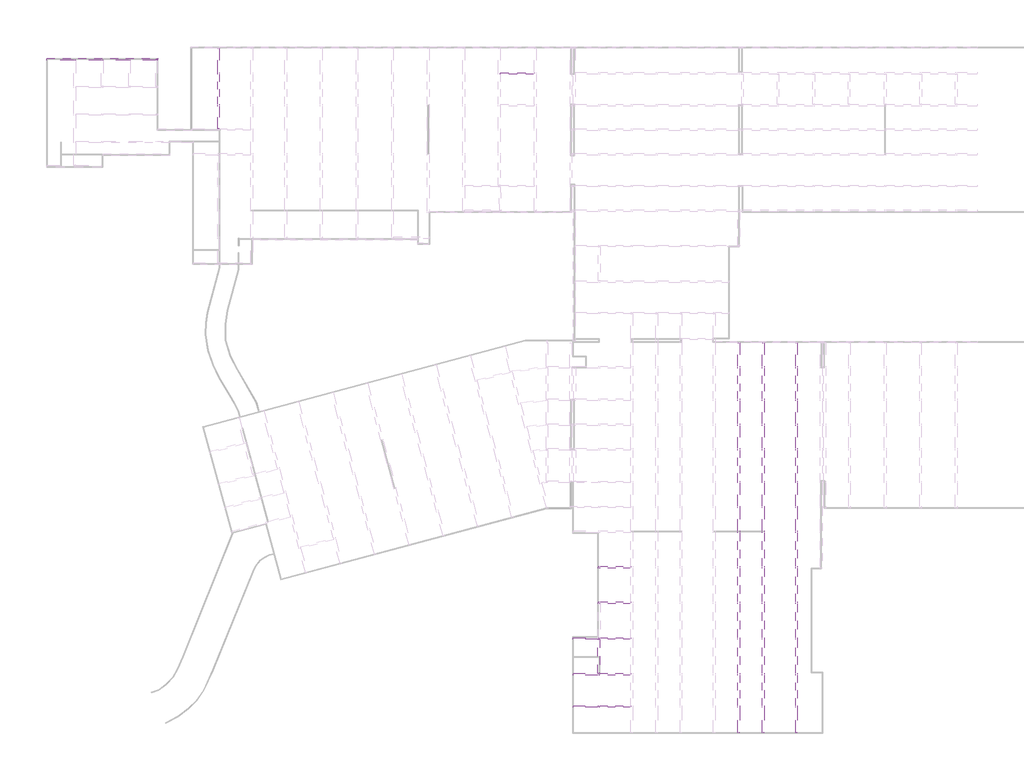
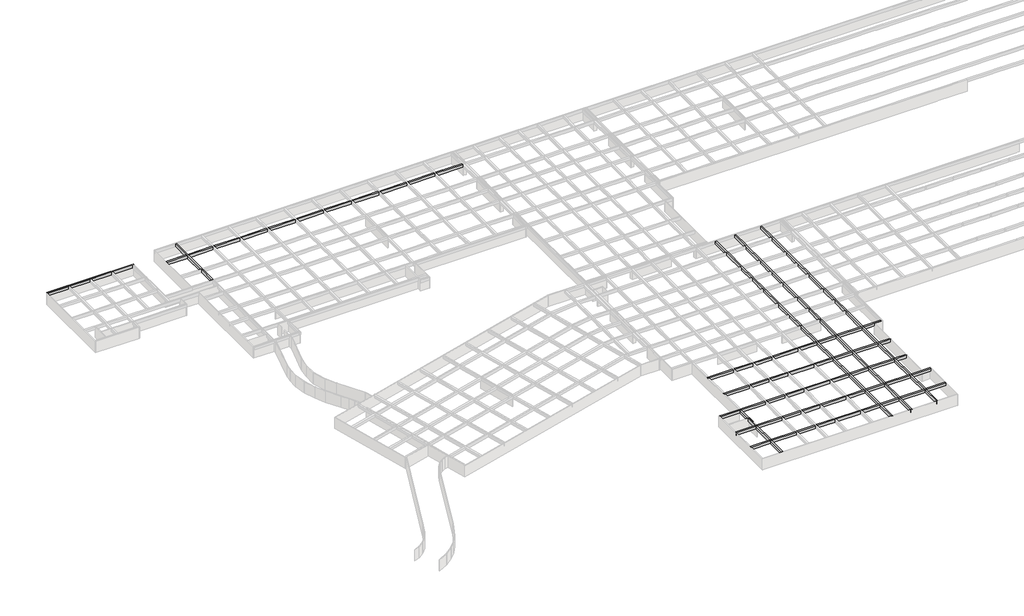
# One storey, part 6 of 14: 12 beams.
"""IFC4 building model written with IfcOpenShell, lengths in millimetres."""

import ifcopenshell
import ifcopenshell.guid

model = None  # the IFC model being written
_history = None  # IfcOwnerHistory: only IFC2X3 demands one
_inside = {}  # id of a spatial element -> (the spatial element, [elements in it])
_under = {}  # id of a project, library or spatial element -> (it, [spatial elements below it])
_declared = {}  # id of a project -> (the project, [libraries it declares])
_typed = {}  # id of a type object -> (the type object, [elements of that type])
_made_of = {}  # id of a material, layer set ... -> (it, [elements and type objects made of it])


def new_model(schema):
    """Start an empty IFC model of exactly this schema.

    Asked for "IFC4X3", IfcOpenShell would pick the latest addendum, in which some entities
    have other attributes; the version numbers below select the first issue.
    IFC2X3 requires an IfcOwnerHistory on every rooted entity: one is made here for all.
    """
    global model, _history
    if schema == "IFC4X3":
        model = ifcopenshell.file(schema_version=(4, 3, 0, 0))
    else:
        model = ifcopenshell.file(schema=schema)
    _inside.clear()
    _under.clear()
    _declared.clear()
    _typed.clear()
    _made_of.clear()
    _history = None
    if model.schema == "IFC2X3":
        org = make("IfcOrganization", Name="unknown")
        user = make(
            "IfcPersonAndOrganization",
            ThePerson=make("IfcPerson", FamilyName="unknown"),
            TheOrganization=org,
        )
        app = make(
            "IfcApplication",
            ApplicationDeveloper=org,
            Version="unknown",
            ApplicationFullName="unknown",
            ApplicationIdentifier="unknown",
        )
        _history = make(
            "IfcOwnerHistory",
            OwningUser=user,
            OwningApplication=app,
            ChangeAction="ADDED",
            CreationDate=0,
        )
    return model


def make(cls, **values):
    """One entity of the class cls with the attributes given. An attribute that is None is left unset."""
    return model.create_entity(
        cls, **{name: value for name, value in values.items() if value is not None}
    )


def rooted(cls, **values):
    """An entity with a GlobalId (a new one), such as an element, a storey or a relation."""
    return make(cls, GlobalId=ifcopenshell.guid.new(), OwnerHistory=_history, **values)


def si_unit(unit_type, name, prefix=None):
    """IfcSIUnit, for example si_unit("LENGTHUNIT", "METRE", prefix="MILLI")."""
    return make("IfcSIUnit", UnitType=unit_type, Prefix=prefix, Name=name)


def assignment(units):
    """IfcUnitAssignment: the units of a project."""
    return None if units is None else make("IfcUnitAssignment", Units=units)


def point(xyz):
    """IfcCartesianPoint."""
    return None if xyz is None else make("IfcCartesianPoint", Coordinates=xyz)


def direction(xyz):
    """IfcDirection."""
    return None if xyz is None else make("IfcDirection", DirectionRatios=xyz)


def frame(location, z_axis=None, x_axis=None):
    """IfcAxis2Placement3D, a coordinate frame: its origin and axes. An axis left out is left unset."""
    return make(
        "IfcAxis2Placement3D",
        Location=point(location),
        Axis=direction(z_axis),
        RefDirection=direction(x_axis),
    )


def origin():
    """The frame at (0, 0, 0) with its axes left unset."""
    return frame((0.0, 0.0, 0.0))


def place(relative_to, where):
    """IfcLocalPlacement: puts the frame where relative to a parent placement (None: the world)."""
    return make(
        "IfcLocalPlacement", PlacementRelTo=relative_to, RelativePlacement=where
    )


def context(
    kind, dimensions, precision=None, world=None, true_north=None, identifier=None
):
    """IfcGeometricRepresentationContext, for example the 3D "Model" context."""
    return make(
        "IfcGeometricRepresentationContext",
        ContextIdentifier=identifier,
        ContextType=kind,
        CoordinateSpaceDimension=dimensions,
        Precision=precision,
        WorldCoordinateSystem=world,
        TrueNorth=true_north,
    )


def project(units=None, contexts=None):
    """IfcProject with its units and contexts."""
    return rooted(
        "IfcProject",
        Name="project",
        RepresentationContexts=contexts,
        UnitsInContext=assignment(units),
    )


def spatial(cls, under=None, at=None, **own):
    """A site, building, storey or space (cls), placed at a placement, below another one or the project."""
    s = rooted(cls, ObjectPlacement=at, **own)
    if under is not None:
        _under.setdefault(under.id(), (under, []))[1].append(s)
    return s


def polyline(points):
    """IfcPolyline through the points."""
    return make("IfcPolyline", Points=[point(p) for p in points])


def outline(outer, holes=None, kind="AREA"):
    """IfcArbitraryClosedProfileDef: a profile drawn as a closed curve; with holes, ...WithVoids."""
    if holes is None:
        return make("IfcArbitraryClosedProfileDef", ProfileType=kind, OuterCurve=outer)
    return make(
        "IfcArbitraryProfileDefWithVoids",
        ProfileType=kind,
        OuterCurve=outer,
        InnerCurves=holes,
    )


def extrude(swept, where, along, depth):
    """IfcExtrudedAreaSolid: the profile swept, set in the frame where, extruded along a direction by depth."""
    return make(
        "IfcExtrudedAreaSolid",
        SweptArea=swept,
        Position=where,
        ExtrudedDirection=direction(along),
        Depth=depth,
    )


def faces_of(points, faces, orient=None, outer=None):
    """IfcFace entities. A face is a list of loops; a loop is a list of indices into points, from 0.

    orient and outer hold one flag for each loop. By default every Orientation is true, the
    first loop of a face is its IfcFaceOuterBound and the others are IfcFaceBound.
    """
    made = []
    for i, loops in enumerate(faces):
        bounds = []
        for j, loop in enumerate(loops):
            is_outer = j == 0 if outer is None else outer[i][j]
            bounds.append(
                make(
                    "IfcFaceOuterBound" if is_outer else "IfcFaceBound",
                    Bound=make("IfcPolyLoop", Polygon=[points[k] for k in loop]),
                    Orientation=True if orient is None else orient[i][j],
                )
            )
        made.append(make("IfcFace", Bounds=bounds))
    return made


def faceted_brep(points, faces, orient=None, outer=None, voids=None):
    """IfcFacetedBrep: a solid bounded by flat faces; with voids (closed shells), ...WithVoids."""
    shared = [point(p) for p in points]
    hull = make("IfcClosedShell", CfsFaces=faces_of(shared, faces, orient, outer))
    if voids is None:
        return make("IfcFacetedBrep", Outer=hull)
    return make(
        "IfcFacetedBrepWithVoids",
        Outer=hull,
        Voids=[
            make(cls, CfsFaces=faces_of(shared, fs, o, b)) for cls, fs, o, b in voids
        ],
    )


def shape(context_of_items, identifier, shape_type, items):
    """IfcShapeRepresentation: the items that make up one representation, for example the "Body"."""
    return make(
        "IfcShapeRepresentation",
        ContextOfItems=context_of_items,
        RepresentationIdentifier=identifier,
        RepresentationType=shape_type,
        Items=items,
    )


def made_of(thing, what):
    """Note that an element or type object is made of a material, layer set ...; save() writes the relation."""
    if what is not None:
        _made_of.setdefault(what.id(), (what, []))[1].append(thing)
    return thing


def element(
    cls,
    number,
    at=None,
    inside=None,
    cuts=None,
    type_object=None,
    material=None,
    context=None,
    identifier="Body",
    shape_type=None,
    held_by="IfcProductDefinitionShape",
    body=None,
    shapes=None,
    **own,
):
    """One element of the class cls, such as IfcWall. Its Tag is "e" and its number.

    at: its placement. inside: the storey or other place that contains it. cuts: it is an
    opening in that element (IfcRelVoidsElement). A single representation is given by context,
    identifier, shape_type and body (its items); several are given by shapes. held_by: the class
    of the entity that holds the representations. save() writes the other relations.
    """
    e = rooted(cls, Tag="e%d" % number, ObjectPlacement=at, **own)
    if body is not None:
        shapes = [shape(context, identifier, shape_type, body)]
    if shapes is not None:
        e.Representation = make(held_by, Representations=shapes)
    if inside is not None:
        _inside.setdefault(inside.id(), (inside, []))[1].append(e)
    if cuts is not None:
        rooted(
            "IfcRelVoidsElement", RelatingBuildingElement=cuts, RelatedOpeningElement=e
        )
    if type_object is not None:
        _typed.setdefault(type_object.id(), (type_object, []))[1].append(e)
    return made_of(e, material)


def aggregate(whole, parts):
    """IfcRelAggregates: a whole, such as a stair, and the parts it consists of."""
    return rooted("IfcRelAggregates", RelatingObject=whole, RelatedObjects=parts)


def save(model, path):
    """Write the relations noted so far, then the file.

    IfcRelAggregates (storeys below a building ...), IfcRelContainedInSpatialStructure (elements
    in a storey), IfcRelDefinesByType, IfcRelAssociatesMaterial and IfcRelDeclares: one each for
    every whole, place, type object, material and project.
    """
    for whole, parts in _under.values():
        aggregate(whole, parts)
    for where, things in _inside.values():
        rooted(
            "IfcRelContainedInSpatialStructure",
            RelatedElements=things,
            RelatingStructure=where,
        )
    for kind, things in _typed.values():
        rooted("IfcRelDefinesByType", RelatedObjects=things, RelatingType=kind)
    for what, things in _made_of.values():
        rooted("IfcRelAssociatesMaterial", RelatedObjects=things, RelatingMaterial=what)
    for by, libraries in _declared.values():
        rooted("IfcRelDeclares", RelatingContext=by, RelatedDefinitions=libraries)
    model.write(path)


model = new_model("IFC4")

# Units and contexts
model_context = context("Model", 3, world=origin())
ifc_project = project(units=[si_unit("LENGTHUNIT", "METRE", prefix="MILLI")], contexts=[model_context])

# Site, building, storey
site = spatial("IfcSite", under=ifc_project)
building = spatial("IfcBuilding", under=site)
storey = spatial("IfcBuildingStorey", under=building, Name="户型图", Elevation=0.0)

# Beams
placement = place(None, origin())
element("IfcBeam", 1, ObjectType="混凝土 - 矩形梁 : KL_beam", at=placement, inside=storey, context=model_context, shape_type="Brep", body=[
    faceted_brep([(-64612.7050956, -135126.4975491, 3300.0), (-64212.7050956, -135126.4975491, 3300.0), (-64212.7050956, -130180.0179086, 3300.0), (-64212.7050956, -129780.0179086, 3300.0), (-64212.7050956, -123258.950757, 3300.0), (-64212.7050956, -122858.950757, 3300.0), (-64212.7050956, -117558.950757, 3300.0), (-64612.7050956, -117558.950757, 3300.0), (-64612.7050956, -122858.950757, 3300.0), (-64612.7050956, -123258.950757, 3300.0), (-64612.7050956, -129780.0179086, 3300.0), (-64612.7050956, -130180.0179086, 3300.0), (-64612.7050956, -135126.4975491, 2500.0), (-64612.7050956, -117558.950757, 2500.0), (-64612.7050956, -122858.950757, 2500.0), (-64612.7050956, -123258.950757, 2500.0), (-64612.7050956, -129780.0179086, 2500.0), (-64612.7050956, -130180.0179086, 2500.0), (-64212.7050956, -135126.4975491, 2500.0), (-64212.7050956, -117558.950757, 2500.0), (-64212.7050956, -122858.950757, 2500.0), (-64212.7050956, -123258.950757, 2500.0), (-64212.7050956, -129780.0179086, 2500.0), (-64212.7050956, -130180.0179086, 2500.0)], [[[0, 1, 2, 3, 4, 5, 6, 7, 8, 9, 10, 11]], [[12, 0, 11, 10, 9, 8, 7, 13, 14, 15, 16, 17]], [[18, 12, 17, 16, 15, 14, 13, 19, 20, 21, 22, 23]], [[1, 18, 23, 22, 21, 20, 19, 6, 5, 4, 3, 2]], [[1, 0, 12, 18]], [[7, 6, 19, 13]]]),
])
element("IfcBeam", 2, ObjectType="混凝土 - 矩形梁 : KL_beam", at=placement, inside=storey, context=model_context, shape_type="SweptSolid", body=[
    extrude(outline(polyline([(-70372.7050956, -123258.950757), (-70372.7050956, -122858.950757), (-64612.7050956, -122858.950757), (-64612.7050956, -123258.950757), (-70372.7050956, -123258.950757)])), frame((0.0, 0.0, 2500.0), z_axis=(0.0, 0.0, 1.0), x_axis=(1.0, 0.0, 0.0)), (0.0, 0.0, 1.0), 800.0),
    extrude(outline(polyline([(-64212.7050956, -123258.950757), (-64212.7050956, -122858.950757), (-57355.3281677, -122858.950757), (-57355.3281677, -123258.950757), (-64212.7050956, -123258.950757)])), frame((0.0, 0.0, 2500.0), z_axis=(0.0, 0.0, 1.0), x_axis=(1.0, 0.0, 0.0)), (0.0, 0.0, 1.0), 800.0),
    extrude(outline(polyline([(12577.2949044, -122858.950757), (12577.2949044, -123258.950757), (5154.7716095, -123258.950757), (5154.7716095, -122858.950757), (12577.2949044, -122858.950757)])), frame((0.0, 0.0, 2500.0), z_axis=(0.0, 0.0, 1.0), x_axis=(1.0, 0.0, 0.0)), (0.0, 0.0, 1.0), 800.0),
    extrude(outline(polyline([(-56955.3281677, -123258.950757), (-56955.3281677, -122858.950757), (-49869.9201432, -122858.950757), (-49869.9201432, -123258.950757), (-56955.3281677, -123258.950757)])), frame((0.0, 0.0, 2500.0), z_axis=(0.0, 0.0, 1.0), x_axis=(1.0, 0.0, 0.0)), (0.0, 0.0, 1.0), 800.0),
    extrude(outline(polyline([(-49469.9201432, -123258.950757), (-49469.9201432, -122858.950757), (-42115.0194088, -122858.950757), (-42115.0194088, -123258.950757), (-49469.9201432, -123258.950757)])), frame((0.0, 0.0, 2500.0), z_axis=(0.0, 0.0, 1.0), x_axis=(1.0, 0.0, 0.0)), (0.0, 0.0, 1.0), 800.0),
    extrude(outline(polyline([(-41715.0194088, -123258.950757), (-41715.0194088, -122858.950757), (-34272.7050956, -122858.950757), (-34272.7050956, -123258.950757), (-41715.0194088, -123258.950757)])), frame((0.0, 0.0, 2500.0), z_axis=(0.0, 0.0, 1.0), x_axis=(1.0, 0.0, 0.0)), (0.0, 0.0, 1.0), 800.0),
    extrude(outline(polyline([(-33872.7050956, -123258.950757), (-33872.7050956, -122858.950757), (-26492.7050956, -122858.950757), (-26492.7050956, -123258.950757), (-33872.7050956, -123258.950757)])), frame((0.0, 0.0, 2500.0), z_axis=(0.0, 0.0, 1.0), x_axis=(1.0, 0.0, 0.0)), (0.0, 0.0, 1.0), 800.0),
    extrude(outline(polyline([(-26092.7050956, -123258.950757), (-26092.7050956, -122858.950757), (-18655.2993912, -122858.950757), (-18655.2993912, -123258.950757), (-26092.7050956, -123258.950757)])), frame((0.0, 0.0, 2500.0), z_axis=(0.0, 0.0, 1.0), x_axis=(1.0, 0.0, 0.0)), (0.0, 0.0, 1.0), 800.0),
    extrude(outline(polyline([(-18255.2993912, -123258.950757), (-18255.2993912, -122858.950757), (-10914.1452268, -122858.950757), (-10914.1452268, -123258.950757), (-18255.2993912, -123258.950757)])), frame((0.0, 0.0, 2500.0), z_axis=(0.0, 0.0, 1.0), x_axis=(1.0, 0.0, 0.0)), (0.0, 0.0, 1.0), 800.0),
    extrude(outline(polyline([(-10514.1452268, -123258.950757), (-10514.1452268, -122858.950757), (-3091.5778774, -122858.950757), (-3091.5778774, -123258.950757), (-10514.1452268, -123258.950757)])), frame((0.0, 0.0, 2500.0), z_axis=(0.0, 0.0, 1.0), x_axis=(1.0, 0.0, 0.0)), (0.0, 0.0, 1.0), 800.0),
    extrude(outline(polyline([(-2691.5778774, -123258.950757), (-2691.5778774, -122858.950757), (4754.7716095, -122858.950757), (4754.7716095, -123258.950757), (-2691.5778774, -123258.950757)])), frame((0.0, 0.0, 2500.0), z_axis=(0.0, 0.0, 1.0), x_axis=(1.0, 0.0, 0.0)), (0.0, 0.0, 1.0), 800.0),
])
element("IfcBeam", 3, ObjectType="混凝土 - 矩形梁 : KL_beam", at=placement, inside=storey, context=model_context, shape_type="Brep", body=[
    faceted_brep([(49689.9831968, -267473.0312098, 3300.0), (49289.9831968, -267473.0312098, 3300.0), (49289.9831968, -267473.0312098, 2500.0), (49689.9831968, -267473.0312098, 2500.0), (49689.9831968, -261891.8929199, 3300.0), (49689.9831968, -261491.8929199, 3300.0), (49689.9831968, -254823.1116625, 3300.0), (49689.9831968, -254423.1116625, 3300.0), (49689.9831968, -247008.950757, 3300.0), (49689.9831968, -246608.950757, 3300.0), (49689.9831968, -239178.950757, 3300.0), (49689.9831968, -238778.950757, 3300.0), (49689.9831968, -231409.1116625, 3300.0), (49689.9831968, -231009.1116625, 3300.0), (49689.9831968, -223621.814057, 3300.0), (49689.9831968, -223221.814057, 3300.0), (49689.9831968, -218208.950757, 3300.0), (49689.9831968, -217808.950757, 3300.0), (49689.9831968, -212708.950757, 3300.0), (49689.9831968, -212308.950757, 3300.0), (49689.9831968, -205576.1028577, 3300.0), (49689.9831968, -205176.1028577, 3300.0), (49689.9831968, -200154.952508, 3300.0), (49689.9831968, -199754.952508, 3300.0), (49689.9831968, -194741.3993539, 3300.0), (49689.9831968, -194341.3993539, 3300.0), (49689.9831968, -187598.950757, 3300.0), (49689.9831968, -187198.950757, 3300.0), (49689.9831968, -182068.950757, 3300.0), (49289.9831968, -182068.950757, 3300.0), (49289.9831968, -187198.950757, 3300.0), (49289.9831968, -187598.950757, 3300.0), (49289.9831968, -194341.3993539, 3300.0), (49289.9831968, -194741.3993539, 3300.0), (49289.9831968, -199754.952508, 3300.0), (49289.9831968, -200154.952508, 3300.0), (49289.9831968, -205176.1028577, 3300.0), (49289.9831968, -205576.1028577, 3300.0), (49289.9831968, -212308.950757, 3300.0), (49289.9831968, -212708.950757, 3300.0), (49289.9831968, -217808.950757, 3300.0), (49289.9831968, -218208.950757, 3300.0), (49289.9831968, -223221.814057, 3300.0), (49289.9831968, -223621.814057, 3300.0), (49289.9831968, -231009.1116625, 3300.0), (49289.9831968, -231409.1116625, 3300.0), (49289.9831968, -238778.950757, 3300.0), (49289.9831968, -239178.950757, 3300.0), (49289.9831968, -246608.950757, 3300.0), (49289.9831968, -247008.950757, 3300.0), (49289.9831968, -254423.1116625, 3300.0), (49289.9831968, -254823.1116625, 3300.0), (49289.9831968, -261491.8929199, 3300.0), (49289.9831968, -261891.8929199, 3300.0), (49289.9831968, -182068.950757, 2500.0), (49289.9831968, -187198.950757, 2500.0), (49289.9831968, -187598.950757, 2500.0), (49289.9831968, -194341.3993539, 2500.0), (49289.9831968, -194741.3993539, 2500.0), (49289.9831968, -199754.952508, 2500.0), (49289.9831968, -200154.952508, 2500.0), (49289.9831968, -205176.1028577, 2500.0), (49289.9831968, -205576.1028577, 2500.0), (49289.9831968, -212308.950757, 2500.0), (49289.9831968, -212708.950757, 2500.0), (49289.9831968, -217808.950757, 2500.0), (49289.9831968, -218208.950757, 2500.0), (49289.9831968, -223221.814057, 2500.0), (49289.9831968, -223621.814057, 2500.0), (49289.9831968, -231009.1116625, 2500.0), (49289.9831968, -231409.1116625, 2500.0), (49289.9831968, -238778.950757, 2500.0), (49289.9831968, -239178.950757, 2500.0), (49289.9831968, -246608.950757, 2500.0), (49289.9831968, -247008.950757, 2500.0), (49289.9831968, -254423.1116625, 2500.0), (49289.9831968, -254823.1116625, 2500.0), (49289.9831968, -261491.8929199, 2500.0), (49289.9831968, -261891.8929199, 2500.0), (49689.9831968, -182068.950757, 2500.0), (49689.9831968, -187198.950757, 2500.0), (49689.9831968, -187598.950757, 2500.0), (49689.9831968, -194341.3993539, 2500.0), (49689.9831968, -194741.3993539, 2500.0), (49689.9831968, -199754.952508, 2500.0), (49689.9831968, -200154.952508, 2500.0), (49689.9831968, -205176.1028577, 2500.0), (49689.9831968, -205576.1028577, 2500.0), (49689.9831968, -212308.950757, 2500.0), (49689.9831968, -212708.950757, 2500.0), (49689.9831968, -217808.950757, 2500.0), (49689.9831968, -218208.950757, 2500.0), (49689.9831968, -223221.814057, 2500.0), (49689.9831968, -223621.814057, 2500.0), (49689.9831968, -231009.1116625, 2500.0), (49689.9831968, -231409.1116625, 2500.0), (49689.9831968, -238778.950757, 2500.0), (49689.9831968, -239178.950757, 2500.0), (49689.9831968, -246608.950757, 2500.0), (49689.9831968, -247008.950757, 2500.0), (49689.9831968, -254423.1116625, 2500.0), (49689.9831968, -254823.1116625, 2500.0), (49689.9831968, -261491.8929199, 2500.0), (49689.9831968, -261891.8929199, 2500.0)], [[[0, 1, 2, 3]], [[1, 0, 4, 5, 6, 7, 8, 9, 10, 11, 12, 13, 14, 15, 16, 17, 18, 19, 20, 21, 22, 23, 24, 25, 26, 27, 28, 29, 30, 31, 32, 33, 34, 35, 36, 37, 38, 39, 40, 41, 42, 43, 44, 45, 46, 47, 48, 49, 50, 51, 52, 53]], [[2, 1, 53, 52, 51, 50, 49, 48, 47, 46, 45, 44, 43, 42, 41, 40, 39, 38, 37, 36, 35, 34, 33, 32, 31, 30, 29, 54, 55, 56, 57, 58, 59, 60, 61, 62, 63, 64, 65, 66, 67, 68, 69, 70, 71, 72, 73, 74, 75, 76, 77, 78]], [[3, 2, 78, 77, 76, 75, 74, 73, 72, 71, 70, 69, 68, 67, 66, 65, 64, 63, 62, 61, 60, 59, 58, 57, 56, 55, 54, 79, 80, 81, 82, 83, 84, 85, 86, 87, 88, 89, 90, 91, 92, 93, 94, 95, 96, 97, 98, 99, 100, 101, 102, 103]], [[0, 3, 103, 102, 101, 100, 99, 98, 97, 96, 95, 94, 93, 92, 91, 90, 89, 88, 87, 86, 85, 84, 83, 82, 81, 80, 79, 28, 27, 26, 25, 24, 23, 22, 21, 20, 19, 18, 17, 16, 15, 14, 13, 12, 11, 10, 9, 8, 7, 6, 5, 4]], [[29, 28, 79, 54]]]),
])
element("IfcBeam", 4, ObjectType="混凝土 - 矩形梁 : KL_beam", at=placement, inside=storey, context=model_context, shape_type="Brep", body=[
    faceted_brep([(54689.9831968, -267473.0312098, 3300.0), (54689.9831968, -267473.0312098, 2500.0), (55089.9831968, -267473.0312098, 2500.0), (55089.9831968, -267473.0312098, 3300.0), (55089.9831968, -261891.8929199, 3300.0), (55089.9831968, -261491.8929199, 3300.0), (55089.9831968, -254823.1116625, 3300.0), (55089.9831968, -254423.1116625, 3300.0), (55089.9831968, -247008.950757, 3300.0), (55089.9831968, -246608.950757, 3300.0), (55089.9831968, -239178.950757, 3300.0), (55089.9831968, -238778.950757, 3300.0), (55089.9831968, -231409.1116625, 3300.0), (55089.9831968, -231009.1116625, 3300.0), (55089.9831968, -223621.814057, 3300.0), (55089.9831968, -223221.814057, 3300.0), (55089.9831968, -218208.950757, 3300.0), (55089.9831968, -217808.950757, 3300.0), (55089.9831968, -212708.950757, 3300.0), (55089.9831968, -212308.950757, 3300.0), (55089.9831968, -205576.1028577, 3300.0), (55089.9831968, -205176.1028577, 3300.0), (55089.9831968, -200154.952508, 3300.0), (55089.9831968, -199754.952508, 3300.0), (55089.9831968, -194741.3993539, 3300.0), (55089.9831968, -194341.3993539, 3300.0), (55089.9831968, -187598.950757, 3300.0), (55089.9831968, -187198.950757, 3300.0), (55089.9831968, -182068.950757, 3300.0), (54689.9831968, -182068.950757, 3300.0), (54689.9831968, -187198.950757, 3300.0), (54689.9831968, -187598.950757, 3300.0), (54689.9831968, -194341.3993539, 3300.0), (54689.9831968, -194741.3993539, 3300.0), (54689.9831968, -199754.952508, 3300.0), (54689.9831968, -200154.952508, 3300.0), (54689.9831968, -205176.1028577, 3300.0), (54689.9831968, -205576.1028577, 3300.0), (54689.9831968, -212308.950757, 3300.0), (54689.9831968, -212708.950757, 3300.0), (54689.9831968, -217808.950757, 3300.0), (54689.9831968, -218208.950757, 3300.0), (54689.9831968, -223221.814057, 3300.0), (54689.9831968, -223621.814057, 3300.0), (54689.9831968, -231009.1116625, 3300.0), (54689.9831968, -231409.1116625, 3300.0), (54689.9831968, -238778.950757, 3300.0), (54689.9831968, -239178.950757, 3300.0), (54689.9831968, -246608.950757, 3300.0), (54689.9831968, -247008.950757, 3300.0), (54689.9831968, -254423.1116625, 3300.0), (54689.9831968, -254823.1116625, 3300.0), (54689.9831968, -261491.8929199, 3300.0), (54689.9831968, -261891.8929199, 3300.0), (55089.9831968, -261891.8929199, 2500.0), (55089.9831968, -261491.8929199, 2500.0), (55089.9831968, -254823.1116625, 2500.0), (55089.9831968, -254423.1116625, 2500.0), (55089.9831968, -247008.950757, 2500.0), (55089.9831968, -246608.950757, 2500.0), (55089.9831968, -239178.950757, 2500.0), (55089.9831968, -238778.950757, 2500.0), (55089.9831968, -231409.1116625, 2500.0), (55089.9831968, -231009.1116625, 2500.0), (55089.9831968, -223621.814057, 2500.0), (55089.9831968, -223221.814057, 2500.0), (55089.9831968, -218208.950757, 2500.0), (55089.9831968, -217808.950757, 2500.0), (55089.9831968, -212708.950757, 2500.0), (55089.9831968, -212308.950757, 2500.0), (55089.9831968, -205576.1028577, 2500.0), (55089.9831968, -205176.1028577, 2500.0), (55089.9831968, -200154.952508, 2500.0), (55089.9831968, -199754.952508, 2500.0), (55089.9831968, -194741.3993539, 2500.0), (55089.9831968, -194341.3993539, 2500.0), (55089.9831968, -187598.950757, 2500.0), (55089.9831968, -187198.950757, 2500.0), (55089.9831968, -182068.950757, 2500.0), (54689.9831968, -261891.8929199, 2500.0), (54689.9831968, -261491.8929199, 2500.0), (54689.9831968, -254823.1116625, 2500.0), (54689.9831968, -254423.1116625, 2500.0), (54689.9831968, -247008.950757, 2500.0), (54689.9831968, -246608.950757, 2500.0), (54689.9831968, -239178.950757, 2500.0), (54689.9831968, -238778.950757, 2500.0), (54689.9831968, -231409.1116625, 2500.0), (54689.9831968, -231009.1116625, 2500.0), (54689.9831968, -223621.814057, 2500.0), (54689.9831968, -223221.814057, 2500.0), (54689.9831968, -218208.950757, 2500.0), (54689.9831968, -217808.950757, 2500.0), (54689.9831968, -212708.950757, 2500.0), (54689.9831968, -212308.950757, 2500.0), (54689.9831968, -205576.1028577, 2500.0), (54689.9831968, -205176.1028577, 2500.0), (54689.9831968, -200154.952508, 2500.0), (54689.9831968, -199754.952508, 2500.0), (54689.9831968, -194741.3993539, 2500.0), (54689.9831968, -194341.3993539, 2500.0), (54689.9831968, -187598.950757, 2500.0), (54689.9831968, -187198.950757, 2500.0), (54689.9831968, -182068.950757, 2500.0)], [[[0, 1, 2, 3]], [[0, 3, 4, 5, 6, 7, 8, 9, 10, 11, 12, 13, 14, 15, 16, 17, 18, 19, 20, 21, 22, 23, 24, 25, 26, 27, 28, 29, 30, 31, 32, 33, 34, 35, 36, 37, 38, 39, 40, 41, 42, 43, 44, 45, 46, 47, 48, 49, 50, 51, 52, 53]], [[3, 2, 54, 55, 56, 57, 58, 59, 60, 61, 62, 63, 64, 65, 66, 67, 68, 69, 70, 71, 72, 73, 74, 75, 76, 77, 78, 28, 27, 26, 25, 24, 23, 22, 21, 20, 19, 18, 17, 16, 15, 14, 13, 12, 11, 10, 9, 8, 7, 6, 5, 4]], [[2, 1, 79, 80, 81, 82, 83, 84, 85, 86, 87, 88, 89, 90, 91, 92, 93, 94, 95, 96, 97, 98, 99, 100, 101, 102, 103, 78, 77, 76, 75, 74, 73, 72, 71, 70, 69, 68, 67, 66, 65, 64, 63, 62, 61, 60, 59, 58, 57, 56, 55, 54]], [[1, 0, 53, 52, 51, 50, 49, 48, 47, 46, 45, 44, 43, 42, 41, 40, 39, 38, 37, 36, 35, 34, 33, 32, 31, 30, 29, 103, 102, 101, 100, 99, 98, 97, 96, 95, 94, 93, 92, 91, 90, 89, 88, 87, 86, 85, 84, 83, 82, 81, 80, 79]], [[29, 28, 78, 103]]]),
])
element("IfcBeam", 5, ObjectType="混凝土 - 矩形梁 : KL_beam", at=placement, inside=storey, context=model_context, shape_type="Brep", body=[
    faceted_brep([(62367.2949044, -267468.950757, 3300.0), (61967.2949044, -267468.950757, 3300.0), (61967.2949044, -267468.950757, 2500.0), (62367.2949044, -267468.950757, 2500.0), (62367.2949044, -261891.8929199, 3300.0), (62367.2949044, -261491.8929199, 3300.0), (62367.2949044, -254823.1116625, 3300.0), (62367.2949044, -254423.1116625, 3300.0), (62367.2949044, -247008.950757, 3300.0), (62367.2949044, -246608.950757, 3300.0), (62367.2949044, -239178.950757, 3300.0), (62367.2949044, -238778.950757, 3300.0), (62367.2949044, -231409.1116625, 3300.0), (62367.2949044, -231009.1116625, 3300.0), (62367.2949044, -223621.814057, 3300.0), (62367.2949044, -223221.814057, 3300.0), (62367.2949044, -218208.950757, 3300.0), (62367.2949044, -217808.950757, 3300.0), (62367.2949044, -212708.950757, 3300.0), (62367.2949044, -212308.950757, 3300.0), (62367.2949044, -205576.1028577, 3300.0), (62367.2949044, -205176.1028577, 3300.0), (62367.2949044, -200154.952508, 3300.0), (62367.2949044, -199754.952508, 3300.0), (62367.2949044, -194741.3993539, 3300.0), (62367.2949044, -194341.3993539, 3300.0), (62367.2949044, -187598.950757, 3300.0), (62367.2949044, -187198.950757, 3300.0), (62367.2949044, -182068.950757, 3300.0), (61967.2949044, -182068.950757, 3300.0), (61967.2949044, -187198.950757, 3300.0), (61967.2949044, -187598.950757, 3300.0), (61967.2949044, -194341.3993539, 3300.0), (61967.2949044, -194741.3993539, 3300.0), (61967.2949044, -199754.952508, 3300.0), (61967.2949044, -200154.952508, 3300.0), (61967.2949044, -205176.1028577, 3300.0), (61967.2949044, -205576.1028577, 3300.0), (61967.2949044, -212308.950757, 3300.0), (61967.2949044, -212708.950757, 3300.0), (61967.2949044, -217808.950757, 3300.0), (61967.2949044, -218208.950757, 3300.0), (61967.2949044, -223221.814057, 3300.0), (61967.2949044, -223621.814057, 3300.0), (61967.2949044, -231009.1116625, 3300.0), (61967.2949044, -231409.1116625, 3300.0), (61967.2949044, -238778.950757, 3300.0), (61967.2949044, -239178.950757, 3300.0), (61967.2949044, -246608.950757, 3300.0), (61967.2949044, -247008.950757, 3300.0), (61967.2949044, -254423.1116625, 3300.0), (61967.2949044, -254823.1116625, 3300.0), (61967.2949044, -261491.8929199, 3300.0), (61967.2949044, -261891.8929199, 3300.0), (61967.2949044, -182068.950757, 2500.0), (61967.2949044, -187198.950757, 2500.0), (61967.2949044, -187598.950757, 2500.0), (61967.2949044, -194341.3993539, 2500.0), (61967.2949044, -194741.3993539, 2500.0), (61967.2949044, -199754.952508, 2500.0), (61967.2949044, -200154.952508, 2500.0), (61967.2949044, -205176.1028577, 2500.0), (61967.2949044, -205576.1028577, 2500.0), (61967.2949044, -212308.950757, 2500.0), (61967.2949044, -212708.950757, 2500.0), (61967.2949044, -217808.950757, 2500.0), (61967.2949044, -218208.950757, 2500.0), (61967.2949044, -223221.814057, 2500.0), (61967.2949044, -223621.814057, 2500.0), (61967.2949044, -231009.1116625, 2500.0), (61967.2949044, -231409.1116625, 2500.0), (61967.2949044, -238778.950757, 2500.0), (61967.2949044, -239178.950757, 2500.0), (61967.2949044, -246608.950757, 2500.0), (61967.2949044, -247008.950757, 2500.0), (61967.2949044, -254423.1116625, 2500.0), (61967.2949044, -254823.1116625, 2500.0), (61967.2949044, -261491.8929199, 2500.0), (61967.2949044, -261891.8929199, 2500.0), (62367.2949044, -182068.950757, 2500.0), (62367.2949044, -187198.950757, 2500.0), (62367.2949044, -187598.950757, 2500.0), (62367.2949044, -194341.3993539, 2500.0), (62367.2949044, -194741.3993539, 2500.0), (62367.2949044, -199754.952508, 2500.0), (62367.2949044, -200154.952508, 2500.0), (62367.2949044, -205176.1028577, 2500.0), (62367.2949044, -205576.1028577, 2500.0), (62367.2949044, -212308.950757, 2500.0), (62367.2949044, -212708.950757, 2500.0), (62367.2949044, -217808.950757, 2500.0), (62367.2949044, -218208.950757, 2500.0), (62367.2949044, -223221.814057, 2500.0), (62367.2949044, -223621.814057, 2500.0), (62367.2949044, -231009.1116625, 2500.0), (62367.2949044, -231409.1116625, 2500.0), (62367.2949044, -238778.950757, 2500.0), (62367.2949044, -239178.950757, 2500.0), (62367.2949044, -246608.950757, 2500.0), (62367.2949044, -247008.950757, 2500.0), (62367.2949044, -254423.1116625, 2500.0), (62367.2949044, -254823.1116625, 2500.0), (62367.2949044, -261491.8929199, 2500.0), (62367.2949044, -261891.8929199, 2500.0)], [[[0, 1, 2, 3]], [[1, 0, 4, 5, 6, 7, 8, 9, 10, 11, 12, 13, 14, 15, 16, 17, 18, 19, 20, 21, 22, 23, 24, 25, 26, 27, 28, 29, 30, 31, 32, 33, 34, 35, 36, 37, 38, 39, 40, 41, 42, 43, 44, 45, 46, 47, 48, 49, 50, 51, 52, 53]], [[2, 1, 53, 52, 51, 50, 49, 48, 47, 46, 45, 44, 43, 42, 41, 40, 39, 38, 37, 36, 35, 34, 33, 32, 31, 30, 29, 54, 55, 56, 57, 58, 59, 60, 61, 62, 63, 64, 65, 66, 67, 68, 69, 70, 71, 72, 73, 74, 75, 76, 77, 78]], [[3, 2, 78, 77, 76, 75, 74, 73, 72, 71, 70, 69, 68, 67, 66, 65, 64, 63, 62, 61, 60, 59, 58, 57, 56, 55, 54, 79, 80, 81, 82, 83, 84, 85, 86, 87, 88, 89, 90, 91, 92, 93, 94, 95, 96, 97, 98, 99, 100, 101, 102, 103]], [[0, 3, 103, 102, 101, 100, 99, 98, 97, 96, 95, 94, 93, 92, 91, 90, 89, 88, 87, 86, 85, 84, 83, 82, 81, 80, 79, 28, 27, 26, 25, 24, 23, 22, 21, 20, 19, 18, 17, 16, 15, 14, 13, 12, 11, 10, 9, 8, 7, 6, 5, 4]], [[29, 28, 79, 54]]]),
])
element("IfcBeam", 6, ObjectType="混凝土 - 矩形梁 : KL_beam", at=placement, inside=storey, context=model_context, shape_type="Brep", body=[
    faceted_brep([(18732.2846424, -231409.1116625, 3300.0), (18732.2846424, -231009.1116625, 3300.0), (18732.2846424, -231009.1116625, 2500.0), (18732.2846424, -231409.1116625, 2500.0), (18760.0865653, -231409.1116625, 3300.0), (19160.0865653, -231409.1116625, 3300.0), (25921.5607309, -231409.1116625, 3300.0), (25921.5607309, -231009.1116625, 3300.0), (19160.0865653, -231009.1116625, 3300.0), (18760.0865653, -231009.1116625, 3300.0), (25921.5607309, -231009.1116625, 2500.0), (19160.0865653, -231009.1116625, 2500.0), (18760.0865653, -231009.1116625, 2500.0), (25921.5607309, -231409.1116625, 2500.0), (19160.0865653, -231409.1116625, 2500.0), (18760.0865653, -231409.1116625, 2500.0)], [[[0, 1, 2, 3]], [[1, 0, 4, 5, 6, 7, 8, 9]], [[2, 1, 9, 8, 7, 10, 11, 12]], [[3, 2, 12, 11, 10, 13, 14, 15]], [[0, 3, 15, 14, 13, 6, 5, 4]], [[7, 6, 13, 10]]]),
    faceted_brep([(67367.2949044, -231009.1116625, 3300.0), (67367.2949044, -231409.1116625, 3300.0), (67367.2949044, -231409.1116625, 2500.0), (67367.2949044, -231009.1116625, 2500.0), (62367.2949044, -231409.1116625, 3300.0), (62367.2949044, -231009.1116625, 3300.0), (62367.2949044, -231009.1116625, 2500.0), (62367.2949044, -231409.1116625, 2500.0)], [[[0, 1, 2, 3]], [[4, 5, 6, 7]], [[1, 0, 5, 4]], [[0, 3, 6, 5]], [[3, 2, 7, 6]], [[2, 1, 4, 7]]]),
    faceted_brep([(26321.5607309, -231409.1116625, 3300.0), (26321.5607309, -231009.1116625, 3300.0), (26321.5607309, -231009.1116625, 2500.0), (26321.5607309, -231409.1116625, 2500.0), (31351.9066405, -231409.1116625, 3300.0), (31351.9066405, -231009.1116625, 3300.0), (31351.9066405, -231009.1116625, 2500.0), (31351.9066405, -231409.1116625, 2500.0)], [[[0, 1, 2, 3]], [[1, 0, 4, 5]], [[2, 1, 5, 6]], [[3, 2, 6, 7]], [[0, 3, 7, 4]], [[5, 4, 7, 6]]]),
    faceted_brep([(31751.9066405, -231409.1116625, 3300.0), (31751.9066405, -231009.1116625, 3300.0), (31751.9066405, -231009.1116625, 2500.0), (31751.9066405, -231409.1116625, 2500.0), (36681.5607309, -231409.1116625, 3300.0), (36681.5607309, -231009.1116625, 3300.0), (36681.5607309, -231009.1116625, 2500.0), (36681.5607309, -231409.1116625, 2500.0)], [[[0, 1, 2, 3]], [[1, 0, 4, 5]], [[2, 1, 5, 6]], [[3, 2, 6, 7]], [[0, 3, 7, 4]], [[5, 4, 7, 6]]]),
    faceted_brep([(37081.5607309, -231409.1116625, 3300.0), (37081.5607309, -231009.1116625, 3300.0), (37081.5607309, -231009.1116625, 2500.0), (37081.5607309, -231409.1116625, 2500.0), (43931.9066405, -231409.1116625, 3300.0), (43931.9066405, -231009.1116625, 3300.0), (43931.9066405, -231009.1116625, 2500.0), (43931.9066405, -231409.1116625, 2500.0)], [[[0, 1, 2, 3]], [[1, 0, 4, 5]], [[2, 1, 5, 6]], [[3, 2, 6, 7]], [[0, 3, 7, 4]], [[5, 4, 7, 6]]]),
    faceted_brep([(44331.9066405, -231409.1116625, 3300.0), (44331.9066405, -231009.1116625, 3300.0), (44331.9066405, -231009.1116625, 2500.0), (44331.9066405, -231409.1116625, 2500.0), (49289.9831968, -231409.1116625, 3300.0), (49289.9831968, -231009.1116625, 3300.0), (49289.9831968, -231009.1116625, 2500.0), (49289.9831968, -231409.1116625, 2500.0)], [[[0, 1, 2, 3]], [[1, 0, 4, 5]], [[2, 1, 5, 6]], [[3, 2, 6, 7]], [[0, 3, 7, 4]], [[5, 4, 7, 6]]]),
    faceted_brep([(49689.9831968, -231409.1116625, 3300.0), (49689.9831968, -231009.1116625, 3300.0), (49689.9831968, -231009.1116625, 2500.0), (49689.9831968, -231409.1116625, 2500.0), (54689.9831968, -231409.1116625, 3300.0), (54689.9831968, -231009.1116625, 3300.0), (54689.9831968, -231009.1116625, 2500.0), (54689.9831968, -231409.1116625, 2500.0)], [[[0, 1, 2, 3]], [[1, 0, 4, 5]], [[2, 1, 5, 6]], [[3, 2, 6, 7]], [[0, 3, 7, 4]], [[5, 4, 7, 6]]]),
    faceted_brep([(55089.9831968, -231409.1116625, 3300.0), (55089.9831968, -231009.1116625, 3300.0), (55089.9831968, -231009.1116625, 2500.0), (55089.9831968, -231409.1116625, 2500.0), (61967.2949044, -231409.1116625, 3300.0), (61967.2949044, -231009.1116625, 3300.0), (61967.2949044, -231009.1116625, 2500.0), (61967.2949044, -231409.1116625, 2500.0)], [[[0, 1, 2, 3]], [[1, 0, 4, 5]], [[2, 1, 5, 6]], [[3, 2, 6, 7]], [[0, 3, 7, 4]], [[5, 4, 7, 6]]]),
])
element("IfcBeam", 7, ObjectType="混凝土 - 矩形梁 : KL_beam", at=placement, inside=storey, context=model_context, shape_type="Brep", body=[
    faceted_brep([(65427.2846424, -238778.950757, 3300.0), (65427.2846424, -239178.950757, 3300.0), (65427.2846424, -239178.950757, 2500.0), (65427.2846424, -238778.950757, 2500.0), (62367.2949044, -238778.950757, 3300.0), (62367.2949044, -239178.950757, 3300.0), (62367.2949044, -239178.950757, 2500.0), (62367.2949044, -238778.950757, 2500.0)], [[[0, 1, 2, 3]], [[1, 0, 4, 5]], [[2, 1, 5, 6]], [[3, 2, 6, 7]], [[0, 3, 7, 4]], [[5, 4, 7, 6]]]),
    faceted_brep([(18732.2846424, -238778.950757, 3300.0), (18732.2846424, -238778.950757, 2500.0), (18732.2846424, -239178.950757, 2500.0), (18732.2846424, -239178.950757, 3300.0), (25921.5607309, -238778.950757, 3300.0), (25921.5607309, -239178.950757, 3300.0), (25921.5607309, -239178.950757, 2500.0), (25921.5607309, -238778.950757, 2500.0), (18760.0865653, -239178.950757, 3300.0), (19160.0865653, -239178.950757, 3300.0), (19160.0865653, -238778.950757, 3300.0), (18760.0865653, -238778.950757, 3300.0), (18760.0865653, -239178.950757, 2500.0), (19160.0865653, -239178.950757, 2500.0), (18760.0865653, -238778.950757, 2500.0), (19160.0865653, -238778.950757, 2500.0)], [[[0, 1, 2, 3]], [[4, 5, 6, 7]], [[0, 3, 8, 9, 5, 4, 10, 11]], [[3, 2, 12, 13, 6, 5, 9, 8]], [[2, 1, 14, 15, 7, 6, 13, 12]], [[1, 0, 11, 10, 4, 7, 15, 14]]]),
    faceted_brep([(26321.5607309, -239178.950757, 3300.0), (26321.5607309, -238778.950757, 3300.0), (26321.5607309, -238778.950757, 2500.0), (26321.5607309, -239178.950757, 2500.0), (31351.9066405, -238778.950757, 3300.0), (31351.9066405, -239178.950757, 3300.0), (31351.9066405, -239178.950757, 2500.0), (31351.9066405, -238778.950757, 2500.0)], [[[0, 1, 2, 3]], [[4, 5, 6, 7]], [[1, 0, 5, 4]], [[0, 3, 6, 5]], [[3, 2, 7, 6]], [[2, 1, 4, 7]]]),
    faceted_brep([(31751.9066405, -239178.950757, 3300.0), (31751.9066405, -238778.950757, 3300.0), (31751.9066405, -238778.950757, 2500.0), (31751.9066405, -239178.950757, 2500.0), (36681.5607309, -238778.950757, 3300.0), (36681.5607309, -239178.950757, 3300.0), (36681.5607309, -239178.950757, 2500.0), (36681.5607309, -238778.950757, 2500.0)], [[[0, 1, 2, 3]], [[4, 5, 6, 7]], [[1, 0, 5, 4]], [[0, 3, 6, 5]], [[3, 2, 7, 6]], [[2, 1, 4, 7]]]),
    faceted_brep([(37081.5607309, -239178.950757, 3300.0), (37081.5607309, -238778.950757, 3300.0), (37081.5607309, -238778.950757, 2500.0), (37081.5607309, -239178.950757, 2500.0), (43931.9066405, -238778.950757, 3300.0), (43931.9066405, -239178.950757, 3300.0), (43931.9066405, -239178.950757, 2500.0), (43931.9066405, -238778.950757, 2500.0)], [[[0, 1, 2, 3]], [[4, 5, 6, 7]], [[1, 0, 5, 4]], [[0, 3, 6, 5]], [[3, 2, 7, 6]], [[2, 1, 4, 7]]]),
    faceted_brep([(44331.9066405, -239178.950757, 3300.0), (44331.9066405, -238778.950757, 3300.0), (44331.9066405, -238778.950757, 2500.0), (44331.9066405, -239178.950757, 2500.0), (49289.9831968, -238778.950757, 3300.0), (49289.9831968, -239178.950757, 3300.0), (49289.9831968, -239178.950757, 2500.0), (49289.9831968, -238778.950757, 2500.0)], [[[0, 1, 2, 3]], [[4, 5, 6, 7]], [[1, 0, 5, 4]], [[0, 3, 6, 5]], [[3, 2, 7, 6]], [[2, 1, 4, 7]]]),
    faceted_brep([(49689.9831968, -239178.950757, 3300.0), (49689.9831968, -238778.950757, 3300.0), (49689.9831968, -238778.950757, 2500.0), (49689.9831968, -239178.950757, 2500.0), (54689.9831968, -238778.950757, 3300.0), (54689.9831968, -239178.950757, 3300.0), (54689.9831968, -239178.950757, 2500.0), (54689.9831968, -238778.950757, 2500.0)], [[[0, 1, 2, 3]], [[4, 5, 6, 7]], [[1, 0, 5, 4]], [[0, 3, 6, 5]], [[3, 2, 7, 6]], [[2, 1, 4, 7]]]),
    faceted_brep([(55089.9831968, -239178.950757, 3300.0), (55089.9831968, -238778.950757, 3300.0), (55089.9831968, -238778.950757, 2500.0), (55089.9831968, -239178.950757, 2500.0), (61967.2949044, -238778.950757, 3300.0), (61967.2949044, -239178.950757, 3300.0), (61967.2949044, -239178.950757, 2500.0), (61967.2949044, -238778.950757, 2500.0)], [[[0, 1, 2, 3]], [[4, 5, 6, 7]], [[1, 0, 5, 4]], [[0, 3, 6, 5]], [[3, 2, 7, 6]], [[2, 1, 4, 7]]]),
])
element("IfcBeam", 8, ObjectType="混凝土 - 矩形梁 : KL_beam", at=placement, inside=storey, context=model_context, shape_type="Brep", body=[
    faceted_brep([(65427.2949044, -246608.950757, 3300.0), (65427.2949044, -247008.950757, 3300.0), (65427.2949044, -247008.950757, 2500.0), (65427.2949044, -246608.950757, 2500.0), (62367.2949044, -246608.950757, 3300.0), (62367.2949044, -247008.950757, 3300.0), (62367.2949044, -247008.950757, 2500.0), (62367.2949044, -246608.950757, 2500.0)], [[[0, 1, 2, 3]], [[1, 0, 4, 5]], [[2, 1, 5, 6]], [[3, 2, 6, 7]], [[0, 3, 7, 4]], [[5, 4, 7, 6]]]),
    faceted_brep([(13227.2949044, -246608.950757, 3300.0), (13227.2949044, -246608.950757, 2500.0), (13227.2949044, -247008.950757, 2500.0), (13227.2949044, -247008.950757, 3300.0), (25921.5607309, -246608.950757, 3300.0), (25921.5607309, -247008.950757, 3300.0), (25921.5607309, -247008.950757, 2500.0), (25921.5607309, -246608.950757, 2500.0), (18677.2949044, -247008.950757, 3300.0), (19077.2949044, -247008.950757, 3300.0), (19160.0865653, -246608.950757, 3300.0), (18760.0865653, -246608.950757, 3300.0), (18677.2949044, -247008.950757, 2500.0), (19077.2949044, -247008.950757, 2500.0), (18760.0865653, -246608.950757, 2500.0), (19160.0865653, -246608.950757, 2500.0)], [[[0, 1, 2, 3]], [[4, 5, 6, 7]], [[0, 3, 8, 9, 5, 4, 10, 11]], [[3, 2, 12, 13, 6, 5, 9, 8]], [[2, 1, 14, 15, 7, 6, 13, 12]], [[1, 0, 11, 10, 4, 7, 15, 14]]]),
    faceted_brep([(26321.5607309, -247008.950757, 3300.0), (26321.5607309, -246608.950757, 3300.0), (26321.5607309, -246608.950757, 2500.0), (26321.5607309, -247008.950757, 2500.0), (31351.9066405, -246608.950757, 3300.0), (31351.9066405, -247008.950757, 3300.0), (31351.9066405, -247008.950757, 2500.0), (31351.9066405, -246608.950757, 2500.0)], [[[0, 1, 2, 3]], [[4, 5, 6, 7]], [[1, 0, 5, 4]], [[0, 3, 6, 5]], [[3, 2, 7, 6]], [[2, 1, 4, 7]]]),
    faceted_brep([(31751.9066405, -247008.950757, 3300.0), (31751.9066405, -246608.950757, 3300.0), (31751.9066405, -246608.950757, 2500.0), (31751.9066405, -247008.950757, 2500.0), (36681.5607309, -246608.950757, 3300.0), (36681.5607309, -247008.950757, 3300.0), (36681.5607309, -247008.950757, 2500.0), (36681.5607309, -246608.950757, 2500.0)], [[[0, 1, 2, 3]], [[4, 5, 6, 7]], [[1, 0, 5, 4]], [[0, 3, 6, 5]], [[3, 2, 7, 6]], [[2, 1, 4, 7]]]),
    faceted_brep([(37081.5607309, -247008.950757, 3300.0), (37081.5607309, -246608.950757, 3300.0), (37081.5607309, -246608.950757, 2500.0), (37081.5607309, -247008.950757, 2500.0), (43931.9066405, -246608.950757, 3300.0), (43931.9066405, -247008.950757, 3300.0), (43931.9066405, -247008.950757, 2500.0), (43931.9066405, -246608.950757, 2500.0)], [[[0, 1, 2, 3]], [[4, 5, 6, 7]], [[1, 0, 5, 4]], [[0, 3, 6, 5]], [[3, 2, 7, 6]], [[2, 1, 4, 7]]]),
    faceted_brep([(44331.9066405, -247008.950757, 3300.0), (44331.9066405, -246608.950757, 3300.0), (44331.9066405, -246608.950757, 2500.0), (44331.9066405, -247008.950757, 2500.0), (49289.9831968, -246608.950757, 3300.0), (49289.9831968, -247008.950757, 3300.0), (49289.9831968, -247008.950757, 2500.0), (49289.9831968, -246608.950757, 2500.0)], [[[0, 1, 2, 3]], [[4, 5, 6, 7]], [[1, 0, 5, 4]], [[0, 3, 6, 5]], [[3, 2, 7, 6]], [[2, 1, 4, 7]]]),
    faceted_brep([(49689.9831968, -247008.950757, 3300.0), (49689.9831968, -246608.950757, 3300.0), (49689.9831968, -246608.950757, 2500.0), (49689.9831968, -247008.950757, 2500.0), (54689.9831968, -246608.950757, 3300.0), (54689.9831968, -247008.950757, 3300.0), (54689.9831968, -247008.950757, 2500.0), (54689.9831968, -246608.950757, 2500.0)], [[[0, 1, 2, 3]], [[4, 5, 6, 7]], [[1, 0, 5, 4]], [[0, 3, 6, 5]], [[3, 2, 7, 6]], [[2, 1, 4, 7]]]),
    faceted_brep([(55089.9831968, -247008.950757, 3300.0), (55089.9831968, -246608.950757, 3300.0), (55089.9831968, -246608.950757, 2500.0), (55089.9831968, -247008.950757, 2500.0), (61967.2949044, -246608.950757, 3300.0), (61967.2949044, -247008.950757, 3300.0), (61967.2949044, -247008.950757, 2500.0), (61967.2949044, -246608.950757, 2500.0)], [[[0, 1, 2, 3]], [[4, 5, 6, 7]], [[1, 0, 5, 4]], [[0, 3, 6, 5]], [[3, 2, 7, 6]], [[2, 1, 4, 7]]]),
])
element("IfcBeam", 9, ObjectType="混凝土 - 矩形梁 : KL_beam", at=placement, inside=storey, context=model_context, shape_type="Brep", body=[
    faceted_brep([(13232.2743803, -254823.1116625, 3300.0), (13232.2743803, -254423.1116625, 3300.0), (13232.2743803, -254423.1116625, 2500.0), (13232.2743803, -254823.1116625, 2500.0), (18677.2949044, -254823.1116625, 3300.0), (19077.2949044, -254823.1116625, 3300.0), (25921.5607309, -254823.1116625, 3300.0), (25921.5607309, -254423.1116625, 3300.0), (19077.2949044, -254423.1116625, 3300.0), (18677.2949044, -254423.1116625, 3300.0), (25921.5607309, -254423.1116625, 2500.0), (19077.2949044, -254423.1116625, 2500.0), (18677.2949044, -254423.1116625, 2500.0), (25921.5607309, -254823.1116625, 2500.0), (19077.2949044, -254823.1116625, 2500.0), (18677.2949044, -254823.1116625, 2500.0)], [[[0, 1, 2, 3]], [[1, 0, 4, 5, 6, 7, 8, 9]], [[2, 1, 9, 8, 7, 10, 11, 12]], [[3, 2, 12, 11, 10, 13, 14, 15]], [[0, 3, 15, 14, 13, 6, 5, 4]], [[7, 6, 13, 10]]]),
    faceted_brep([(67832.2743803, -254823.1116625, 3300.0), (67832.2743803, -254823.1116625, 2500.0), (67832.2743803, -254423.1116625, 2500.0), (67832.2743803, -254423.1116625, 3300.0), (62367.2949044, -254823.1116625, 3300.0), (62367.2949044, -254423.1116625, 3300.0), (62367.2949044, -254423.1116625, 2500.0), (62367.2949044, -254823.1116625, 2500.0)], [[[0, 1, 2, 3]], [[4, 5, 6, 7]], [[0, 3, 5, 4]], [[3, 2, 6, 5]], [[2, 1, 7, 6]], [[1, 0, 4, 7]]]),
    faceted_brep([(26321.5607309, -254823.1116625, 3300.0), (26321.5607309, -254423.1116625, 3300.0), (26321.5607309, -254423.1116625, 2500.0), (26321.5607309, -254823.1116625, 2500.0), (31351.9066405, -254823.1116625, 3300.0), (31351.9066405, -254423.1116625, 3300.0), (31351.9066405, -254423.1116625, 2500.0), (31351.9066405, -254823.1116625, 2500.0)], [[[0, 1, 2, 3]], [[1, 0, 4, 5]], [[2, 1, 5, 6]], [[3, 2, 6, 7]], [[0, 3, 7, 4]], [[5, 4, 7, 6]]]),
    faceted_brep([(31751.9066405, -254823.1116625, 3300.0), (31751.9066405, -254423.1116625, 3300.0), (31751.9066405, -254423.1116625, 2500.0), (31751.9066405, -254823.1116625, 2500.0), (36681.5607309, -254823.1116625, 3300.0), (36681.5607309, -254423.1116625, 3300.0), (36681.5607309, -254423.1116625, 2500.0), (36681.5607309, -254823.1116625, 2500.0)], [[[0, 1, 2, 3]], [[1, 0, 4, 5]], [[2, 1, 5, 6]], [[3, 2, 6, 7]], [[0, 3, 7, 4]], [[5, 4, 7, 6]]]),
    faceted_brep([(37081.5607309, -254823.1116625, 3300.0), (37081.5607309, -254423.1116625, 3300.0), (37081.5607309, -254423.1116625, 2500.0), (37081.5607309, -254823.1116625, 2500.0), (43931.9066405, -254823.1116625, 3300.0), (43931.9066405, -254423.1116625, 3300.0), (43931.9066405, -254423.1116625, 2500.0), (43931.9066405, -254823.1116625, 2500.0)], [[[0, 1, 2, 3]], [[1, 0, 4, 5]], [[2, 1, 5, 6]], [[3, 2, 6, 7]], [[0, 3, 7, 4]], [[5, 4, 7, 6]]]),
    faceted_brep([(44331.9066405, -254823.1116625, 3300.0), (44331.9066405, -254423.1116625, 3300.0), (44331.9066405, -254423.1116625, 2500.0), (44331.9066405, -254823.1116625, 2500.0), (49289.9831968, -254823.1116625, 3300.0), (49289.9831968, -254423.1116625, 3300.0), (49289.9831968, -254423.1116625, 2500.0), (49289.9831968, -254823.1116625, 2500.0)], [[[0, 1, 2, 3]], [[1, 0, 4, 5]], [[2, 1, 5, 6]], [[3, 2, 6, 7]], [[0, 3, 7, 4]], [[5, 4, 7, 6]]]),
    faceted_brep([(49689.9831968, -254823.1116625, 3300.0), (49689.9831968, -254423.1116625, 3300.0), (49689.9831968, -254423.1116625, 2500.0), (49689.9831968, -254823.1116625, 2500.0), (54689.9831968, -254823.1116625, 3300.0), (54689.9831968, -254423.1116625, 3300.0), (54689.9831968, -254423.1116625, 2500.0), (54689.9831968, -254823.1116625, 2500.0)], [[[0, 1, 2, 3]], [[1, 0, 4, 5]], [[2, 1, 5, 6]], [[3, 2, 6, 7]], [[0, 3, 7, 4]], [[5, 4, 7, 6]]]),
    faceted_brep([(55089.9831968, -254823.1116625, 3300.0), (55089.9831968, -254423.1116625, 3300.0), (55089.9831968, -254423.1116625, 2500.0), (55089.9831968, -254823.1116625, 2500.0), (61967.2949044, -254823.1116625, 3300.0), (61967.2949044, -254423.1116625, 3300.0), (61967.2949044, -254423.1116625, 2500.0), (61967.2949044, -254823.1116625, 2500.0)], [[[0, 1, 2, 3]], [[1, 0, 4, 5]], [[2, 1, 5, 6]], [[3, 2, 6, 7]], [[0, 3, 7, 4]], [[5, 4, 7, 6]]]),
])
element("IfcBeam", 10, ObjectType="混凝土 - 矩形梁 : KL_beam", at=placement, inside=storey, context=model_context, shape_type="Brep", body=[
    faceted_brep([(67832.2743803, -261491.8929199, 3300.0), (67832.2743803, -261891.8929199, 3300.0), (67832.2743803, -261891.8929199, 2500.0), (67832.2743803, -261491.8929199, 2500.0), (62367.2949044, -261491.8929199, 3300.0), (62367.2949044, -261891.8929199, 3300.0), (62367.2949044, -261891.8929199, 2500.0), (62367.2949044, -261491.8929199, 2500.0)], [[[0, 1, 2, 3]], [[1, 0, 4, 5]], [[2, 1, 5, 6]], [[3, 2, 6, 7]], [[0, 3, 7, 4]], [[5, 4, 7, 6]]]),
    faceted_brep([(13232.2743803, -261491.8929199, 3300.0), (13232.2743803, -261491.8929199, 2500.0), (13232.2743803, -261891.8929199, 2500.0), (13232.2743803, -261891.8929199, 3300.0), (25921.5607309, -261491.8929199, 3300.0), (25921.5607309, -261891.8929199, 3300.0), (25921.5607309, -261891.8929199, 2500.0), (25921.5607309, -261491.8929199, 2500.0), (18677.2949044, -261891.8929199, 3300.0), (19077.2949044, -261891.8929199, 3300.0), (19077.2949044, -261491.8929199, 3300.0), (18677.2949044, -261491.8929199, 3300.0), (18677.2949044, -261891.8929199, 2500.0), (19077.2949044, -261891.8929199, 2500.0), (18677.2949044, -261491.8929199, 2500.0), (19077.2949044, -261491.8929199, 2500.0)], [[[0, 1, 2, 3]], [[4, 5, 6, 7]], [[0, 3, 8, 9, 5, 4, 10, 11]], [[3, 2, 12, 13, 6, 5, 9, 8]], [[2, 1, 14, 15, 7, 6, 13, 12]], [[1, 0, 11, 10, 4, 7, 15, 14]]]),
    faceted_brep([(26321.5607309, -261891.8929199, 3300.0), (26321.5607309, -261491.8929199, 3300.0), (26321.5607309, -261491.8929199, 2500.0), (26321.5607309, -261891.8929199, 2500.0), (31351.9066405, -261491.8929199, 3300.0), (31351.9066405, -261891.8929199, 3300.0), (31351.9066405, -261891.8929199, 2500.0), (31351.9066405, -261491.8929199, 2500.0)], [[[0, 1, 2, 3]], [[4, 5, 6, 7]], [[1, 0, 5, 4]], [[0, 3, 6, 5]], [[3, 2, 7, 6]], [[2, 1, 4, 7]]]),
    faceted_brep([(31751.9066405, -261891.8929199, 3300.0), (31751.9066405, -261491.8929199, 3300.0), (31751.9066405, -261491.8929199, 2500.0), (31751.9066405, -261891.8929199, 2500.0), (36681.5607309, -261491.8929199, 3300.0), (36681.5607309, -261891.8929199, 3300.0), (36681.5607309, -261891.8929199, 2500.0), (36681.5607309, -261491.8929199, 2500.0)], [[[0, 1, 2, 3]], [[4, 5, 6, 7]], [[1, 0, 5, 4]], [[0, 3, 6, 5]], [[3, 2, 7, 6]], [[2, 1, 4, 7]]]),
    faceted_brep([(37081.5607309, -261891.8929199, 3300.0), (37081.5607309, -261491.8929199, 3300.0), (37081.5607309, -261491.8929199, 2500.0), (37081.5607309, -261891.8929199, 2500.0), (43931.9066405, -261491.8929199, 3300.0), (43931.9066405, -261891.8929199, 3300.0), (43931.9066405, -261891.8929199, 2500.0), (43931.9066405, -261491.8929199, 2500.0)], [[[0, 1, 2, 3]], [[4, 5, 6, 7]], [[1, 0, 5, 4]], [[0, 3, 6, 5]], [[3, 2, 7, 6]], [[2, 1, 4, 7]]]),
    faceted_brep([(44331.9066405, -261891.8929199, 3300.0), (44331.9066405, -261491.8929199, 3300.0), (44331.9066405, -261491.8929199, 2500.0), (44331.9066405, -261891.8929199, 2500.0), (49289.9831968, -261491.8929199, 3300.0), (49289.9831968, -261891.8929199, 3300.0), (49289.9831968, -261891.8929199, 2500.0), (49289.9831968, -261491.8929199, 2500.0)], [[[0, 1, 2, 3]], [[4, 5, 6, 7]], [[1, 0, 5, 4]], [[0, 3, 6, 5]], [[3, 2, 7, 6]], [[2, 1, 4, 7]]]),
    faceted_brep([(49689.9831968, -261891.8929199, 3300.0), (49689.9831968, -261491.8929199, 3300.0), (49689.9831968, -261491.8929199, 2500.0), (49689.9831968, -261891.8929199, 2500.0), (54689.9831968, -261491.8929199, 3300.0), (54689.9831968, -261891.8929199, 3300.0), (54689.9831968, -261891.8929199, 2500.0), (54689.9831968, -261491.8929199, 2500.0)], [[[0, 1, 2, 3]], [[4, 5, 6, 7]], [[1, 0, 5, 4]], [[0, 3, 6, 5]], [[3, 2, 7, 6]], [[2, 1, 4, 7]]]),
    faceted_brep([(55089.9831968, -261891.8929199, 3300.0), (55089.9831968, -261491.8929199, 3300.0), (55089.9831968, -261491.8929199, 2500.0), (55089.9831968, -261891.8929199, 2500.0), (61967.2949044, -261491.8929199, 3300.0), (61967.2949044, -261891.8929199, 3300.0), (61967.2949044, -261891.8929199, 2500.0), (61967.2949044, -261491.8929199, 2500.0)], [[[0, 1, 2, 3]], [[4, 5, 6, 7]], [[1, 0, 5, 4]], [[0, 3, 6, 5]], [[3, 2, 7, 6]], [[2, 1, 4, 7]]]),
])
element("IfcBeam", 11, ObjectType="混凝土 - 矩形梁 : KL_beam", at=placement, inside=storey, context=model_context, shape_type="SweptSolid", body=[
    extrude(outline(polyline([(19077.2949044, -267208.950757), (18677.2949044, -267208.950757), (18677.2949044, -261891.8929199), (19077.2949044, -261891.8929199), (19077.2949044, -267208.950757)])), frame((0.0, 0.0, 2500.0), z_axis=(0.0, 0.0, 1.0), x_axis=(1.0, 0.0, 0.0)), (0.0, 0.0, 1.0), 800.0),
    extrude(outline(polyline([(18677.2949044, -247008.950757), (19077.2949044, -247008.950757), (19077.2949044, -254423.1116625), (18677.2949044, -254423.1116625), (18677.2949044, -247008.950757)])), frame((0.0, 0.0, 2500.0), z_axis=(0.0, 0.0, 1.0), x_axis=(1.0, 0.0, 0.0)), (0.0, 0.0, 1.0), 800.0),
    extrude(outline(polyline([(18677.2949044, -254823.1116625), (19077.2949044, -254823.1116625), (19077.2949044, -261491.8929199), (18677.2949044, -261491.8929199), (18677.2949044, -254823.1116625)])), frame((0.0, 0.0, 2500.0), z_axis=(0.0, 0.0, 1.0), x_axis=(1.0, 0.0, 0.0)), (0.0, 0.0, 1.0), 800.0),
])
element("IfcBeam", 12, ObjectType="混凝土 - 矩形梁 : KL_beam", at=placement, inside=storey, context=model_context, shape_type="Brep", body=[
    faceted_brep([(-77750.8485237, -119734.1750557, 3300.0), (-77750.8485237, -120134.1750557, 3300.0), (-77750.8485237, -120134.1750557, 2500.0), (-77750.8485237, -119734.1750557, 2500.0), (-102000.8485237, -119734.1750557, 3300.0), (-102000.8485237, -119734.1750557, 2500.0), (-102000.8485237, -120134.1750557, 2500.0), (-102000.8485237, -120134.1750557, 3300.0), (-96064.0025134, -120134.1750557, 3300.0), (-95664.0025134, -120134.1750557, 3300.0), (-90075.8485237, -120134.1750557, 3300.0), (-89675.8485237, -120134.1750557, 3300.0), (-84075.8485237, -120134.1750557, 3300.0), (-83675.8485237, -120134.1750557, 3300.0), (-78200.8485237, -120134.1750557, 3300.0), (-78200.8485237, -119934.6304265, 3300.0), (-77800.8485237, -119934.6304265, 3300.0), (-77800.8485237, -120134.1750557, 3300.0), (-77800.8485237, -120134.1750557, 2500.0), (-77800.8485237, -119934.6304265, 2500.0), (-78200.8485237, -119934.6304265, 2500.0), (-78200.8485237, -120134.1750557, 2500.0), (-83675.8485237, -120134.1750557, 2500.0), (-84075.8485237, -120134.1750557, 2500.0), (-89675.8485237, -120134.1750557, 2500.0), (-90075.8485237, -120134.1750557, 2500.0), (-95664.0025134, -120134.1750557, 2500.0), (-96064.0025134, -120134.1750557, 2500.0)], [[[0, 1, 2, 3]], [[4, 5, 6, 7]], [[1, 0, 4, 7, 8, 9, 10, 11, 12, 13, 14, 15, 16, 17]], [[2, 1, 17, 18]], [[3, 2, 18, 19, 20, 21, 22, 23, 24, 25, 26, 27, 6, 5]], [[0, 3, 5, 4]], [[19, 16, 15, 20]], [[16, 19, 18, 17]], [[20, 15, 14, 21]], [[7, 6, 27, 26, 25, 24, 23, 22, 21, 14, 13, 12, 11, 10, 9, 8]]]),
])

save(model, "model.ifc")

# Revit data of these elements
# Type "混凝土 - 矩形梁 : KL_beam"
#   Length [instance default] = 1524 mm
#   b = 400 mm
#   h = 800 mm
#   Structural Material [instance default] = 混凝土 - 现场浇注混凝土
#   Assembly Code = ""
# Elements 1, 2, 3, 4, 5, 6, 7, 8, 9, 10, 11, 12 (IfcBeam, "混凝土 - 矩形梁 : KL_beam")
#   Comments = ""
#   Structural Material = none
#   Phase Created = 新构造
# Materials
#   "混凝土 - 现场浇注混凝土": class "混凝土", colour RGB 192 192 192, transparency 0
